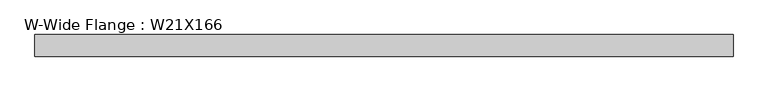
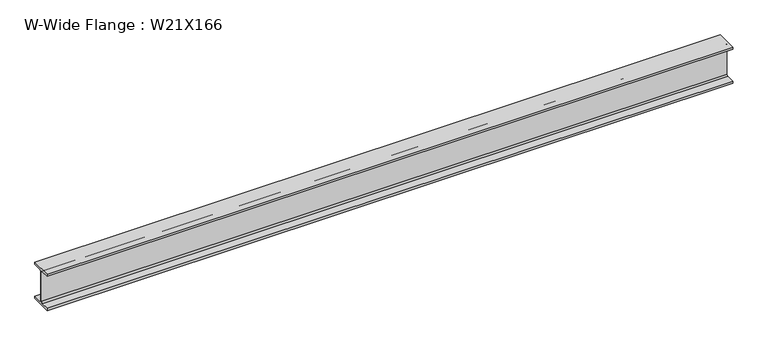
"""IFC4 building model written with IfcOpenShell, lengths in millimetres: beam geometry, W-Wide Flange : W21X166."""

import ifcopenshell
import ifcopenshell.guid

model = None  # the IFC model being written
_history = None  # IfcOwnerHistory: only IFC2X3 demands one
_inside = {}  # id of a spatial element -> (the spatial element, [elements in it])
_under = {}  # id of a project, library or spatial element -> (it, [spatial elements below it])
_declared = {}  # id of a project -> (the project, [libraries it declares])
_typed = {}  # id of a type object -> (the type object, [elements of that type])
_made_of = {}  # id of a material, layer set ... -> (it, [elements and type objects made of it])


def new_model(schema):
    """Start an empty IFC model of exactly this schema.

    Asked for "IFC4X3", IfcOpenShell would pick the latest addendum, in which some entities
    have other attributes; the version numbers below select the first issue.
    IFC2X3 requires an IfcOwnerHistory on every rooted entity: one is made here for all.
    """
    global model, _history
    if schema == "IFC4X3":
        model = ifcopenshell.file(schema_version=(4, 3, 0, 0))
    else:
        model = ifcopenshell.file(schema=schema)
    _inside.clear()
    _under.clear()
    _declared.clear()
    _typed.clear()
    _made_of.clear()
    _history = None
    if model.schema == "IFC2X3":
        org = make("IfcOrganization", Name="unknown")
        user = make(
            "IfcPersonAndOrganization",
            ThePerson=make("IfcPerson", FamilyName="unknown"),
            TheOrganization=org,
        )
        app = make(
            "IfcApplication",
            ApplicationDeveloper=org,
            Version="unknown",
            ApplicationFullName="unknown",
            ApplicationIdentifier="unknown",
        )
        _history = make(
            "IfcOwnerHistory",
            OwningUser=user,
            OwningApplication=app,
            ChangeAction="ADDED",
            CreationDate=0,
        )
    return model


def make(cls, **values):
    """One entity of the class cls with the attributes given. An attribute that is None is left unset."""
    return model.create_entity(
        cls, **{name: value for name, value in values.items() if value is not None}
    )


def rooted(cls, **values):
    """An entity with a GlobalId (a new one), such as an element, a storey or a relation."""
    return make(cls, GlobalId=ifcopenshell.guid.new(), OwnerHistory=_history, **values)


def si_unit(unit_type, name, prefix=None):
    """IfcSIUnit, for example si_unit("LENGTHUNIT", "METRE", prefix="MILLI")."""
    return make("IfcSIUnit", UnitType=unit_type, Prefix=prefix, Name=name)


def assignment(units):
    """IfcUnitAssignment: the units of a project."""
    return None if units is None else make("IfcUnitAssignment", Units=units)


def point(xyz):
    """IfcCartesianPoint."""
    return None if xyz is None else make("IfcCartesianPoint", Coordinates=xyz)


def direction(xyz):
    """IfcDirection."""
    return None if xyz is None else make("IfcDirection", DirectionRatios=xyz)


def frame(location, z_axis=None, x_axis=None):
    """IfcAxis2Placement3D, a coordinate frame: its origin and axes. An axis left out is left unset."""
    return make(
        "IfcAxis2Placement3D",
        Location=point(location),
        Axis=direction(z_axis),
        RefDirection=direction(x_axis),
    )


def frame_2d(location, x_axis=None):
    """IfcAxis2Placement2D, a coordinate frame in the plane: its origin and x axis."""
    return make(
        "IfcAxis2Placement2D", Location=point(location), RefDirection=direction(x_axis)
    )


def origin():
    """The frame at (0, 0, 0) with its axes left unset."""
    return frame((0.0, 0.0, 0.0))


def place(relative_to, where):
    """IfcLocalPlacement: puts the frame where relative to a parent placement (None: the world)."""
    return make(
        "IfcLocalPlacement", PlacementRelTo=relative_to, RelativePlacement=where
    )


def context(
    kind, dimensions, precision=None, world=None, true_north=None, identifier=None
):
    """IfcGeometricRepresentationContext, for example the 3D "Model" context."""
    return make(
        "IfcGeometricRepresentationContext",
        ContextIdentifier=identifier,
        ContextType=kind,
        CoordinateSpaceDimension=dimensions,
        Precision=precision,
        WorldCoordinateSystem=world,
        TrueNorth=true_north,
    )


def project(units=None, contexts=None):
    """IfcProject with its units and contexts."""
    return rooted(
        "IfcProject",
        Name="project",
        RepresentationContexts=contexts,
        UnitsInContext=assignment(units),
    )


def spatial(cls, under=None, at=None, **own):
    """A site, building, storey or space (cls), placed at a placement, below another one or the project."""
    s = rooted(cls, ObjectPlacement=at, **own)
    if under is not None:
        _under.setdefault(under.id(), (under, []))[1].append(s)
    return s


def polyline(points):
    """IfcPolyline through the points."""
    return make("IfcPolyline", Points=[point(p) for p in points])


def circle_curve(where, radius):
    """IfcCircle in the frame where."""
    return make("IfcCircle", Position=where, Radius=radius)


def trimmed(basis, trim1, trim2, sense, master):
    """IfcTrimmedCurve: the piece of a basis curve between two trims."""
    return make(
        "IfcTrimmedCurve",
        BasisCurve=basis,
        Trim1=trim1,
        Trim2=trim2,
        SenseAgreement=sense,
        MasterRepresentation=master,
    )


def segment(curve, same_sense, transition):
    """IfcCompositeCurveSegment."""
    return make(
        "IfcCompositeCurveSegment",
        Transition=transition,
        SameSense=same_sense,
        ParentCurve=curve,
    )


def composite_curve(segments, self_intersect=None):
    """IfcCompositeCurve: segments joined end to end."""
    return make("IfcCompositeCurve", Segments=segments, SelfIntersect=self_intersect)


def outline(outer, holes=None, kind="AREA"):
    """IfcArbitraryClosedProfileDef: a profile drawn as a closed curve; with holes, ...WithVoids."""
    if holes is None:
        return make("IfcArbitraryClosedProfileDef", ProfileType=kind, OuterCurve=outer)
    return make(
        "IfcArbitraryProfileDefWithVoids",
        ProfileType=kind,
        OuterCurve=outer,
        InnerCurves=holes,
    )


def extrude(swept, where, along, depth):
    """IfcExtrudedAreaSolid: the profile swept, set in the frame where, extruded along a direction by depth."""
    return make(
        "IfcExtrudedAreaSolid",
        SweptArea=swept,
        Position=where,
        ExtrudedDirection=direction(along),
        Depth=depth,
    )


def shape(context_of_items, identifier, shape_type, items):
    """IfcShapeRepresentation: the items that make up one representation, for example the "Body"."""
    return make(
        "IfcShapeRepresentation",
        ContextOfItems=context_of_items,
        RepresentationIdentifier=identifier,
        RepresentationType=shape_type,
        Items=items,
    )


def source(mapping_origin, context_of_items, identifier, shape_type, items):
    """IfcRepresentationMap: a shape defined once, which mapped items show again and again."""
    return make(
        "IfcRepresentationMap",
        MappingOrigin=mapping_origin,
        MappedRepresentation=shape(context_of_items, identifier, shape_type, items),
    )


def transform(
    local_origin,
    x_axis=None,
    y_axis=None,
    z_axis=None,
    scale=None,
    scale2=None,
    scale3=None,
    uniform=True,
):
    """IfcCartesianTransformationOperator3D, or its non-uniform kind. x_axis, y_axis, z_axis: its Axis1, 2, 3."""
    if uniform:
        return make(
            "IfcCartesianTransformationOperator3D",
            Axis1=direction(x_axis),
            Axis2=direction(y_axis),
            LocalOrigin=point(local_origin),
            Scale=scale,
            Axis3=direction(z_axis),
        )
    return make(
        "IfcCartesianTransformationOperator3DnonUniform",
        Axis1=direction(x_axis),
        Axis2=direction(y_axis),
        LocalOrigin=point(local_origin),
        Scale=scale,
        Axis3=direction(z_axis),
        Scale2=scale2,
        Scale3=scale3,
    )


def mapped(mapping_source, mapping_target):
    """IfcMappedItem: shows the shape of a source again, moved by a transform."""
    return make(
        "IfcMappedItem", MappingSource=mapping_source, MappingTarget=mapping_target
    )


def made_of(thing, what):
    """Note that an element or type object is made of a material, layer set ...; save() writes the relation."""
    if what is not None:
        _made_of.setdefault(what.id(), (what, []))[1].append(thing)
    return thing


def element(
    cls,
    number,
    at=None,
    inside=None,
    cuts=None,
    type_object=None,
    material=None,
    context=None,
    identifier="Body",
    shape_type=None,
    held_by="IfcProductDefinitionShape",
    body=None,
    shapes=None,
    **own,
):
    """One element of the class cls, such as IfcWall. Its Tag is "e" and its number.

    at: its placement. inside: the storey or other place that contains it. cuts: it is an
    opening in that element (IfcRelVoidsElement). A single representation is given by context,
    identifier, shape_type and body (its items); several are given by shapes. held_by: the class
    of the entity that holds the representations. save() writes the other relations.
    """
    e = rooted(cls, Tag="e%d" % number, ObjectPlacement=at, **own)
    if body is not None:
        shapes = [shape(context, identifier, shape_type, body)]
    if shapes is not None:
        e.Representation = make(held_by, Representations=shapes)
    if inside is not None:
        _inside.setdefault(inside.id(), (inside, []))[1].append(e)
    if cuts is not None:
        rooted(
            "IfcRelVoidsElement", RelatingBuildingElement=cuts, RelatedOpeningElement=e
        )
    if type_object is not None:
        _typed.setdefault(type_object.id(), (type_object, []))[1].append(e)
    return made_of(e, material)


def aggregate(whole, parts):
    """IfcRelAggregates: a whole, such as a stair, and the parts it consists of."""
    return rooted("IfcRelAggregates", RelatingObject=whole, RelatedObjects=parts)


def save(model, path):
    """Write the relations noted so far, then the file.

    IfcRelAggregates (storeys below a building ...), IfcRelContainedInSpatialStructure (elements
    in a storey), IfcRelDefinesByType, IfcRelAssociatesMaterial and IfcRelDeclares: one each for
    every whole, place, type object, material and project.
    """
    for whole, parts in _under.values():
        aggregate(whole, parts)
    for where, things in _inside.values():
        rooted(
            "IfcRelContainedInSpatialStructure",
            RelatedElements=things,
            RelatingStructure=where,
        )
    for kind, things in _typed.values():
        rooted("IfcRelDefinesByType", RelatedObjects=things, RelatingType=kind)
    for what, things in _made_of.values():
        rooted("IfcRelAssociatesMaterial", RelatedObjects=things, RelatingMaterial=what)
    for by, libraries in _declared.values():
        rooted("IfcRelDeclares", RelatingContext=by, RelatedDefinitions=libraries)
    model.write(path)


def w_wide_flange_w21x166_82cd9a53(model_context):
    return source(origin(), model_context, "Body", "SweptSolid", [
        extrude(outline(composite_curve([segment(polyline([(157.48, -251.206), (157.48, -285.75), (-157.48, -285.75), (-157.48, -251.206), (-32.131, -251.206)]), True, "CONTINUOUS"), segment(trimmed(circle_curve(frame_2d((-32.131, -228.6)), 22.606), [point((-32.131, -251.206))], [point((-9.525, -228.6))], True, "CARTESIAN"), True, "CONTINUOUS"), segment(polyline([(-9.525, -228.6), (-9.525, 228.6)]), True, "CONTINUOUS"), segment(trimmed(circle_curve(frame_2d((-32.131, 228.6)), 22.606), [point((-9.525, 228.6))], [point((-32.131, 251.206))], True, "CARTESIAN"), True, "CONTINUOUS"), segment(polyline([(-32.131, 251.206), (-157.48, 251.206), (-157.48, 285.75), (157.48, 285.75), (157.48, 251.206), (32.131, 251.206)]), True, "CONTINUOUS"), segment(trimmed(circle_curve(frame_2d((32.131, 228.6)), 22.606), [point((32.131, 251.206))], [point((9.525, 228.6))], True, "CARTESIAN"), True, "CONTINUOUS"), segment(polyline([(9.525, 228.6), (9.525, -228.6)]), True, "CONTINUOUS"), segment(trimmed(circle_curve(frame_2d((32.131, -228.6)), 22.606), [point((9.525, -228.6))], [point((32.131, -251.206))], True, "CARTESIAN"), True, "CONTINUOUS"), segment(polyline([(32.131, -251.206), (157.48, -251.206)]), True, "CONTINUOUS")], self_intersect=False)), frame((-5180.0235462, 0.0, 0.0), z_axis=(1.0, 0.0, 0.0), x_axis=(0.0, 1.0, 0.0)), (0.0, 0.0, 1.0), 10182.9648149),
    ])


if __name__ == "__main__":
    model = new_model("IFC4")
    model_context = context("Model", 3, world=origin())
    ifc_project = project(units=[si_unit("LENGTHUNIT", "METRE", prefix="MILLI")], contexts=[model_context])
    site = spatial("IfcSite", under=ifc_project)
    building = spatial("IfcBuilding", under=site)
    placement = place(None, origin())
    w_wide_flange_w21x166_shape = w_wide_flange_w21x166_82cd9a53(model_context)
    element("IfcBeam", 1, ObjectType="W-Wide Flange : W21X166", at=placement, inside=building, context=model_context, shape_type="MappedRepresentation", body=[
        mapped(w_wide_flange_w21x166_shape, transform((0.0, 0.0, 0.0), x_axis=(1.0, 0.0, 0.0), y_axis=(0.0, 1.0, 0.0), z_axis=(0.0, 0.0, 1.0))),
    ])
    save(model, "model.ifc")

# Revit data of these elements
# Type "W-Wide Flange : W21X166"
#   Assembly Code = "B10"
#   W = 166
#   Length [instance default] = 5' - 0"
#   bf = 1' - 0.4"
#   d = 1' - 10 1/2"
#   k = 0' - 2 1/4"
#   k2 = 0' - 0.89"
#   tf = 0' - 1.36"
#   tw = 0' - 0 3/4"
#   A = 0.338889 SF
#   Structural Material [instance default] = Steel ASTM A992
# Element 1 (IfcBeam, "W-Wide Flange : W21X166")
#   Materials on its faces: "Steel ASTM A992"
# Materials
#   "Steel ASTM A992": class "Metal", colour RGB 199 199 199, transparency 0, Description = "Structural steel 50ksi", Cost = 0
